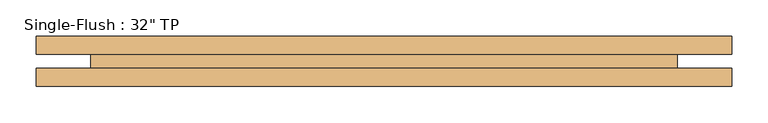
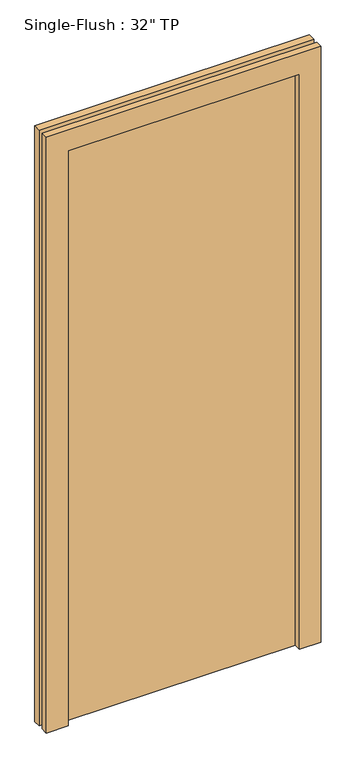
"""IFC4 building model written with IfcOpenShell, lengths in millimetres: door geometry."""

from ifc_helpers import new_model, si_unit, frame, origin, origin_with_axes, place, context, project, spatial, polyline, outline, extrude, source, transform, mapped, element, save


def door_b5082e26(model_context):
    return source(origin(), model_context, "Body", "SweptSolid", [
        extrude(outline(polyline([(2209.8, -482.6), (0.0, -482.6), (0.0, -406.4), (2133.6, -406.4), (2133.6, 406.4), (0.0, 406.4), (0.0, 482.6), (2209.8, 482.6), (2209.8, -482.6)])), frame((0.0, 9.525, 0.0), z_axis=(0.0, 1.0, 0.0), x_axis=(0.0, 0.0, 1.0)), (0.0, 0.0, 1.0), 25.4),
        extrude(outline(polyline([(2209.8, 482.6), (2209.8, -482.6), (0.0, -482.6), (0.0, -406.4), (2133.6, -406.4), (2133.6, 406.4), (0.0, 406.4), (0.0, 482.6), (2209.8, 482.6)])), frame((0.0, -34.925, 0.0), z_axis=(0.0, 1.0, 0.0), x_axis=(0.0, 0.0, 1.0)), (0.0, 0.0, 1.0), 25.4),
        extrude(outline(polyline([(406.4, -9.525), (-406.4, -9.525), (-406.4, 9.525), (406.4, 9.525), (406.4, -9.525)])), origin_with_axes(), (0.0, 0.0, 1.0), 2133.6),
    ])


if __name__ == "__main__":
    model = new_model("IFC4")
    model_context = context("Model", 3, world=origin())
    ifc_project = project(units=[si_unit("LENGTHUNIT", "METRE", prefix="MILLI")], contexts=[model_context])
    site = spatial("IfcSite", under=ifc_project)
    building = spatial("IfcBuilding", under=site)
    placement = place(None, origin())
    door_shape = door_b5082e26(model_context)
    element("IfcDoor", 1, ObjectType="Single-Flush : 32\" TP", at=placement, inside=building, context=model_context, shape_type="MappedRepresentation", body=[
        mapped(door_shape, transform((0.0, 0.0, 0.0), x_axis=(1.0, 0.0, 0.0), y_axis=(0.0, 1.0, 0.0), z_axis=(0.0, 0.0, 1.0))),
    ])
    save(model, "model.ifc")

# Revit data of these elements
# Type "Single-Flush : 32\" TP"
#   Type Mark = "58"
#   Construction Type Id = "MDOOR"
#   Assembly Code = "C1020"
#   Analytic Construction = "Metal"
#   Thickness = 0' - 0 3/4"
#   Heat Transfer Coefficient (U) = 3.7021 W/(m²·K)
#   Height = 7' - 0"
#   Trim Projection Ext = 0' - 1"
#   Trim Projection Int = 0' - 1"
#   Trim Width = 0' - 3"
#   Width = 2' - 8"
#   Door Material = Door - Panel
#   Frame Material = Door - Frame
#   Visual Light Transmittance = 0
#   Solar Heat Gain Coefficient = 0
#   Function = (empty or 0)
#   Wall Closure = (empty or 0)
# Element 1 (IfcDoor, "Single-Flush : 32\" TP")
#   Materials on its faces: "Door - Frame", "Door - Panel"
# Materials
#   "Door - Panel": class "Wood", colour RGB 210 159 95, transparency 0
#   "Door - Frame": class "Miscellaneous", colour RGB 118 70 51, transparency 0
